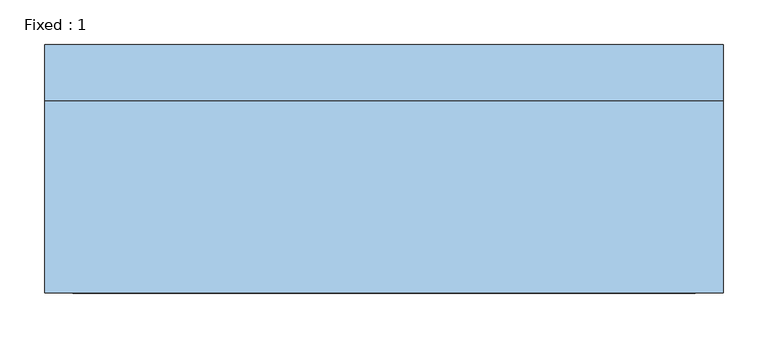
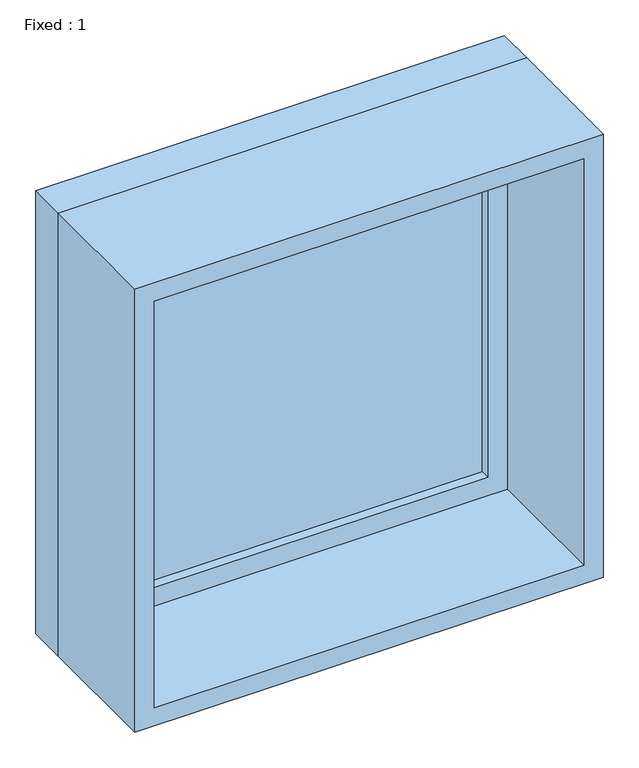
"""IFC4 building model written with IfcOpenShell, lengths in millimetres: window geometry, Fixed : 1."""

from ifc_helpers import new_model, si_unit, frame, origin, place, context, project, spatial, polyline, outline, extrude, source, transform, mapped, element, save


def fixed_1_cc56f13b(model_context):
    return source(origin(), model_context, "Body", "SweptSolid", [
        extrude(outline(polyline([(279.4, 92.075), (-355.6, 92.075), (-355.6, 104.775), (279.4, 104.775), (279.4, 92.075)])), frame((0.0, 0.0, 977.9), z_axis=(0.0, 0.0, 1.0), x_axis=(1.0, 0.0, 0.0)), (0.0, 0.0, 1.0), 635.0),
        extrude(outline(polyline([(1657.35, -400.05), (933.45, -400.05), (933.45, 323.85), (1657.35, 323.85), (1657.35, -400.05)]), holes=[polyline([(1612.9, -355.6), (1612.9, 279.4), (977.9, 279.4), (977.9, -355.6), (1612.9, -355.6)])]), frame((0.0, 76.2, 0.0), z_axis=(0.0, 1.0, 0.0), x_axis=(0.0, 0.0, 1.0)), (0.0, 0.0, 1.0), 44.45),
        extrude(outline(polyline([(1676.4, -419.1), (914.4, -419.1), (914.4, 342.9), (1676.4, 342.9), (1676.4, -419.1)]), holes=[polyline([(1644.65, -387.35), (1644.65, 311.15), (946.15, 311.15), (946.15, -387.35), (1644.65, -387.35)])]), frame((0.0, -139.7, 0.0), z_axis=(0.0, 1.0, 0.0), x_axis=(0.0, 0.0, 1.0)), (0.0, 0.0, 1.0), 215.9),
        extrude(outline(polyline([(1676.4, 342.9), (1676.4, -419.1), (914.4, -419.1), (914.4, 342.9), (1676.4, 342.9)]), holes=[polyline([(1657.35, 323.85), (933.45, 323.85), (933.45, -400.05), (1657.35, -400.05), (1657.35, 323.85)])]), frame((0.0, 76.2, 0.0), z_axis=(0.0, 1.0, 0.0), x_axis=(0.0, 0.0, 1.0)), (0.0, 0.0, 1.0), 63.5),
    ])


if __name__ == "__main__":
    model = new_model("IFC4")
    model_context = context("Model", 3, world=origin())
    ifc_project = project(units=[si_unit("LENGTHUNIT", "METRE", prefix="MILLI")], contexts=[model_context])
    site = spatial("IfcSite", under=ifc_project)
    building = spatial("IfcBuilding", under=site)
    placement = place(None, origin())
    fixed_1_shape = fixed_1_cc56f13b(model_context)
    element("IfcWindow", 1, ObjectType="Fixed : 1", at=placement, inside=building, context=model_context, shape_type="MappedRepresentation", body=[
        mapped(fixed_1_shape, transform((0.0, 0.0, 0.0), x_axis=(1.0, 0.0, 0.0), y_axis=(0.0, 1.0, 0.0), z_axis=(0.0, 0.0, 1.0))),
    ])
    save(model, "model.ifc")

# Revit data of these elements
# Type "Fixed : 1"
#   Type Mark = "11"
#   Assembly Code = "B2020100"
#   Height = 2' - 6"
#   Default Sill Height = 3' - 0"
#   Width = 2' - 6"
#   Window Inset = 0' - 0 3/4"
#   Glass Pane Material = Glass
#   Sash Material = accent 1
#   Wall Closure = (empty or 0)
# Element 1 (IfcWindow, "Fixed : 1")
#   Materials on its faces: "accent 1", "Glass"
# Materials
#   "Glass": class "Glass", colour RGB 236 240 239, transparency 0.85, Description = "Soda Lime Glass", Cost = 0
#   "accent 1": class "Generic", colour RGB 92 104 51, transparency 0, Cost = 0
